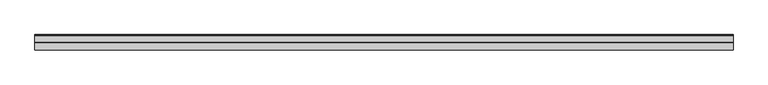
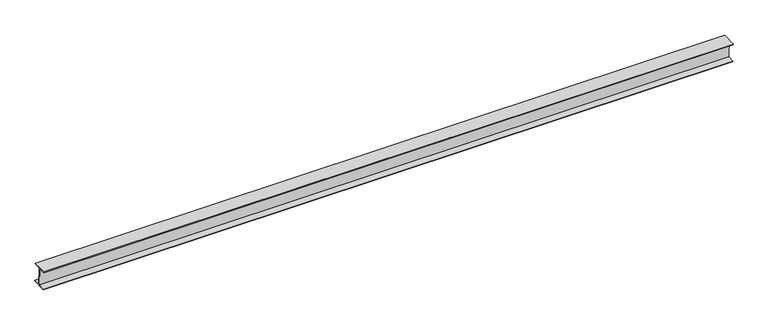
"""IFC4 building model written with IfcOpenShell, lengths in millimetres: proxy geometry, Generic Models 7:Generic Models 1:8:Generic Models 1:8 : Generic Models 7:Generic Models 1:337419:25 : Generic Models 7:Generic Models 1:8:Generic Models 1:8 : Generic Models 7:Generic Models 1:337419:315935."""

from ifc_helpers import new_model, si_unit, frame, origin, place, context, project, spatial, polyline, outline, extrude, source, transform, mapped, element, save


def generic_models_5e798851(model_context):
    return source(origin(), model_context, "Body", "SweptSolid", [
        extrude(outline(polyline([(-565009.8071826, 8903.8547483), (-565010.0795913, 8910.707336), (-564857.7998658, 8916.7608623), (-564857.5274571, 8909.9082746), (-564930.7486251, 8906.9975374), (-564923.2220741, 8717.6630786), (-564850.0193695, 8720.5730819), (-564849.7469608, 8713.7204942), (-565002.0266864, 8707.6669679), (-565002.2990951, 8714.5195556), (-564929.3132631, 8717.4209376), (-564936.8398142, 8906.7553964), (-565009.8071826, 8903.8547483)])), frame((588867.6367242, 0.0, 0.0), z_axis=(1.0, 0.0, 0.0), x_axis=(0.0, 1.0, 0.0)), (0.0, 0.0, 1.0), 7315.2),
    ])


if __name__ == "__main__":
    model = new_model("IFC4")
    model_context = context("Model", 3, world=origin())
    ifc_project = project(units=[si_unit("LENGTHUNIT", "METRE", prefix="MILLI")], contexts=[model_context])
    site = spatial("IfcSite", under=ifc_project)
    building = spatial("IfcBuilding", under=site)
    placement = place(None, origin())
    generic_models_shape = generic_models_5e798851(model_context)
    element("IfcBuildingElementProxy", 1, Name="Generic Models 7:Generic Models 1:8:Generic Models 1:8 : Generic Models 7:Generic Models 1:337419:25 : Generic Models 7:Generic Models 1:8:Generic Models 1:8 : Generic Models 7:Generic Models 1:337419:315935", ObjectType="Generic Models 7:Generic Models 1:8:Generic Models 1:8 : Generic Models 7:Generic Models 1:337419:25 : Generic Models 7:Generic Models 1:8:Generic Models 1:8 : Generic Models 7:Generic Models 1:337419:315935", at=placement, inside=building, context=model_context, shape_type="MappedRepresentation", body=[
        mapped(generic_models_shape, transform((0.0, 0.0, 0.0), x_axis=(1.0, 0.0, 0.0), y_axis=(0.0, 1.0, 0.0), z_axis=(0.0, 0.0, 1.0))),
    ])
    save(model, "model.ifc")

# Revit data of these elements
# Type "Generic Models 7:Generic Models 1:8:Generic Models 1:8 : Generic Models 7:Generic Models 1:337419:25 : Generic Models 7:Generic Models 1:8:Generic Models 1:8 : Generic Models 7:Generic Models 1:337419:315935"
#   NameOverride = "Generic Models 7:Generic Models 1:8:Generic Models 1:8 : Generic Models 7:Generic Models 1:337419:315935"
#   ObjectTypeOverride = "Generic Models 1:8 : Generic Models 7:Generic Models 1:337419"
#   Reference = "Generic Models 1"
#   Tag = "315935"
# Element 1 (IfcBuildingElementProxy, "Generic Models 7:Generic Models 1:8:Generic Models 1:8 : Generic Models 7:Generic Models 1:337419:25 : Generic Models 7:Generic Models 1:8:Generic Models 1:8 : Generic Models 7:Generic Models 1:337419:315935")
#   Materials on its faces: "STRUCTURAL STEEL - SEE STRUCT. DWGS"
# Materials
#   "STRUCTURAL STEEL - SEE STRUCT. DWGS": class "Metal", colour RGB 189 187 185, transparency 0, Description = "Structural steel 50ksi", Cost = 0
